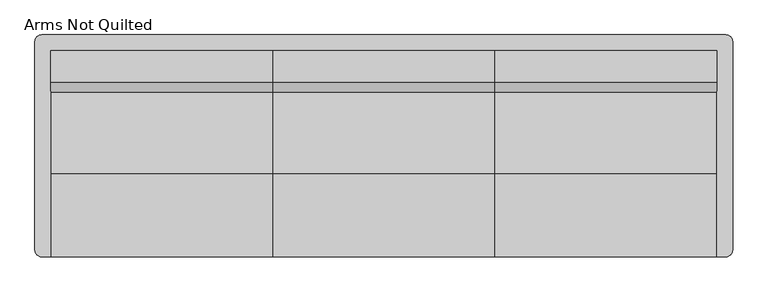
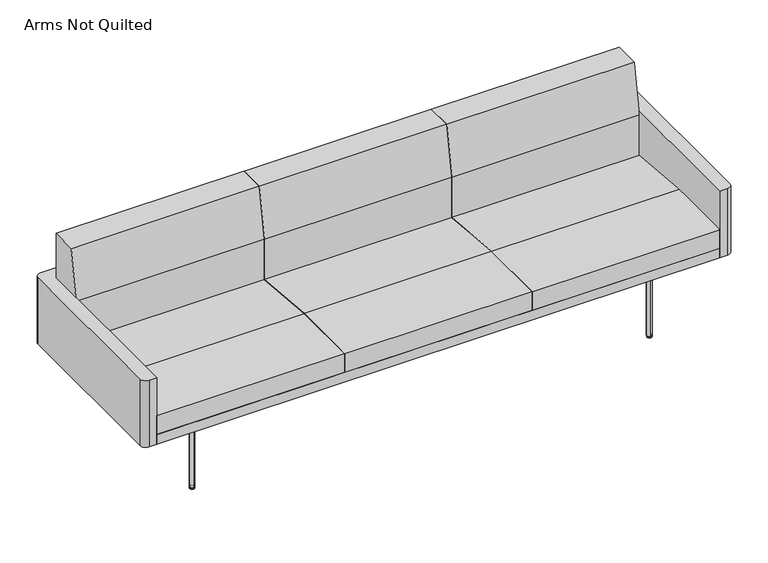
"""IFC4 building model written with IfcOpenShell, lengths in millimetres: furniture geometry, HermanMiller_Collection_Tuxedo_Sofa : Arms Not Quilted."""

from ifc_helpers import new_model, si_unit, point, frame, frame_2d, origin, place, context, project, spatial, polyline, circle_curve, ellipse_curve, trimmed, segment, composite_curve, outline, extrude, source, transform, mapped, element, save
from ifc_brep_helpers import plane_surface, revolved_surface, advanced_brep


def arms_not_quilted_5b6e58a6(model_context):
    return source(origin(), model_context, "Body", "SolidModel", [
        extrude(outline(polyline([(172.790312, 570.0407405), (204.8303749, 761.9999879), (305.047338, 761.9999879), (305.047338, 357.1875), (172.790312, 357.1875), (172.790312, 570.0407405)])), frame((355.8486449, 0.0, 0.0), z_axis=(1.0, 0.0, 0.0), x_axis=(0.0, 1.0, 0.0)), (0.0, 0.0, 1.0), 711.3174324),
        extrude(outline(polyline([(204.8303749, 761.9999879), (305.047338, 761.9999879), (305.047338, 357.1875), (172.790312, 357.1875), (172.790312, 570.0407405), (204.8303749, 761.9999879)])), frame((-1067.1660773, 0.0, 0.0), z_axis=(1.0, 0.0, 0.0), x_axis=(0.0, 1.0, 0.0)), (0.0, 0.0, 1.0), 711.3174324),
        extrude(outline(polyline([(172.790312, 570.0407405), (204.8303749, 761.9999879), (305.047338, 761.9999879), (305.047338, 357.1875), (172.790312, 357.1875), (172.790312, 570.0407405)])), frame((-354.5786449, 0.0, 0.0), z_axis=(1.0, 0.0, 0.0), x_axis=(0.0, 1.0, 0.0)), (0.0, 0.0, 1.0), 709.1572898),
        extrude(outline(polyline([(-355.847338, 357.1875), (-355.847338, 431.3641497), (-89.4717005, 431.3641497), (172.790312, 408.4192229), (172.790312, 357.1875), (-355.847338, 357.1875)])), frame((355.8486449, 0.0, 0.0), z_axis=(1.0, 0.0, 0.0), x_axis=(0.0, 1.0, 0.0)), (0.0, 0.0, 1.0), 711.3174324),
        extrude(outline(polyline([(-355.847338, 431.3641497), (-89.4717005, 431.3641497), (172.790312, 408.4192229), (172.790312, 357.1875), (-355.847338, 357.1875), (-355.847338, 431.3641497)])), frame((-1067.1660773, 0.0, 0.0), z_axis=(1.0, 0.0, 0.0), x_axis=(0.0, 1.0, 0.0)), (0.0, 0.0, 1.0), 711.3174324),
        extrude(outline(polyline([(-355.847338, 357.1875), (-355.847338, 431.3641497), (-89.4717005, 431.3641497), (172.790312, 408.4192229), (172.790312, 357.1875), (-355.847338, 357.1875)])), frame((-354.5786449, 0.0, 0.0), z_axis=(1.0, 0.0, 0.0), x_axis=(0.0, 1.0, 0.0)), (0.0, 0.0, 1.0), 709.1572898),
        advanced_brep(
        [(-862.2241883, -239.6951247, 0.0), (-869.7905542, -239.6951247, 0.0), (-866.0073712, -239.6951247, 0.0), (-856.4823712, -239.6951247, 3.1750001), (-875.5323712, -239.6951247, 3.1750001), (-856.351925, -239.6951247, 6.4931848), (-875.6628174, -239.6951247, 6.4931848), (-861.8574966, -239.6951247, 9.5049435), (-870.1572459, -239.6951247, 9.5049435), (-866.0073712, -239.6951247, 9.5049435)],
        [
            (0, 1, circle_curve(frame((-866.0073712, -239.6951247, 0.0), z_axis=(0.0, 0.0, -1.0), x_axis=(-1.0, 0.0, 0.0)), 3.783183)),
            (1, 2),
            (2, 0),
            (1, 0, circle_curve(frame((-866.0073712, -239.6951247, 0.0), z_axis=(0.0, 0.0, -1.0), x_axis=(-1.0, 0.0, 0.0)), 3.783183)),
            (3, 4, circle_curve(frame((-866.0073712, -239.6951247, 3.1750001), z_axis=(0.0, 0.0, -1.0), x_axis=(-1.0, 0.0, 0.0)), 9.525)),
            (4, 1, circle_curve(frame((-869.7905542, -239.6951247, 6.7793838), z_axis=(0.0, -1.0, 0.0), x_axis=(-1.0, 0.0, 0.0)), 6.7793838)),
            (0, 3, circle_curve(frame((-862.2241883, -239.6951247, 6.7793838), z_axis=(0.0, -1.0, 0.0), x_axis=(1.0, 0.0, 0.0)), 6.7793838)),
            (4, 3, circle_curve(frame((-866.0073712, -239.6951247, 3.1750001), z_axis=(0.0, 0.0, -1.0), x_axis=(-1.0, 0.0, 0.0)), 9.525)),
            (5, 6, circle_curve(frame((-866.0073712, -239.6951247, 6.4931848), z_axis=(0.0, 0.0, -1.0), x_axis=(-1.0, 0.0, 0.0)), 9.6554462)),
            (6, 4),
            (3, 5),
            (6, 5, circle_curve(frame((-866.0073712, -239.6951247, 6.4931848), z_axis=(0.0, 0.0, -1.0), x_axis=(-1.0, 0.0, 0.0)), 9.6554462)),
            (7, 8, circle_curve(frame((-866.0073712, -239.6951247, 9.5049435), z_axis=(0.0, 0.0, -1.0), x_axis=(-1.0, 0.0, 0.0)), 4.1498747)),
            (8, 6, circle_curve(frame((-870.1572459, -239.6951247, 2.9669016), z_axis=(0.0, -1.0, 0.0), x_axis=(-1.0, 0.0, 0.0)), 6.5380418)),
            (5, 7, circle_curve(frame((-861.8574966, -239.6951247, 2.9669016), z_axis=(0.0, -1.0, 0.0), x_axis=(1.0, 0.0, 0.0)), 6.5380418)),
            (8, 7, circle_curve(frame((-866.0073712, -239.6951247, 9.5049435), z_axis=(0.0, 0.0, -1.0), x_axis=(-1.0, 0.0, 0.0)), 4.1498747)),
            (9, 8),
            (7, 9),
        ],
        [
            plane_surface(frame((-866.0073712, -239.6951247, 0.0), z_axis=(0.0, 0.0, -1.0), x_axis=(-1.0, 0.0, 0.0))),
            revolved_surface(trimmed(ellipse_curve(frame((-869.7905542, -239.6951247, 6.7793838), z_axis=(0.0, 1.0, 0.0), x_axis=(-1.0, 0.0, 0.0)), 6.7793838, 6.7793838), [point((-869.7905542, -239.6951247, 0.0))], [point((-875.5323712, -239.6951247, 3.1750001))], True, "CARTESIAN"), (-866.0073712, -239.6951247, 2.4865786), (0.0, 0.0, 1.0)),
            revolved_surface(polyline([(-875.5323712, -239.6951247, 3.1750001), (-875.6628174, -239.6951247, 6.4931848)]), (-866.0073712, -239.6951247, 2.4865786), (0.0, 0.0, 1.0)),
            revolved_surface(trimmed(ellipse_curve(frame((-870.1572459, -239.6951247, 2.9669016), z_axis=(0.0, 1.0, 0.0), x_axis=(-1.0, 0.0, 0.0)), 6.5380418, 6.5380418), [point((-875.6628174, -239.6951247, 6.4931848))], [point((-870.1572459, -239.6951247, 9.5049435))], True, "CARTESIAN"), (-866.0073712, -239.6951247, 2.4865786), (0.0, 0.0, 1.0)),
            plane_surface(frame((-866.0073712, -239.6951247, 9.5049435), z_axis=(0.0, 0.0, 1.0), x_axis=(-1.0, 0.0, 0.0))),
        ],
        [
            (0, [[1, 2, 3]]),
            (0, [[4, -3, -2]]),
            (1, [[5, 6, -1, 7]]),
            (1, [[8, -7, -4, -6]]),
            (2, [[9, 10, -5, 11]]),
            (2, [[12, -11, -8, -10]]),
            (3, [[13, 14, -9, 15]]),
            (3, [[16, -15, -12, -14]]),
            (4, [[17, -13, 18]]),
            (4, [[-18, -16, -17]]),
        ],
    ),
        advanced_brep(
        [(-866.0073712, 332.5700088, 0.0), (-869.7905542, 332.5700088, 0.0), (-862.2241883, 332.5700088, 0.0), (-875.5323712, 332.5700088, 3.1750001), (-856.4823712, 332.5700088, 3.1750001), (-875.6628174, 332.5700088, 6.4931848), (-856.351925, 332.5700088, 6.4931848), (-870.1572459, 332.5700088, 9.5049435), (-861.8574966, 332.5700088, 9.5049435), (-866.0073712, 332.5700088, 9.5049435)],
        [
            (0, 1),
            (1, 2, circle_curve(frame((-866.0073712, 332.5700088, 0.0), z_axis=(0.0, 0.0, -1.0), x_axis=(-1.0, 0.0, 0.0)), 3.783183)),
            (2, 0),
            (2, 1, circle_curve(frame((-866.0073712, 332.5700088, 0.0), z_axis=(0.0, 0.0, -1.0), x_axis=(-1.0, 0.0, 0.0)), 3.783183)),
            (1, 3, circle_curve(frame((-869.7905542, 332.5700088, 6.7793838), z_axis=(0.0, 1.0, 0.0), x_axis=(-1.0, 0.0, 0.0)), 6.7793838)),
            (3, 4, circle_curve(frame((-866.0073712, 332.5700088, 3.1750001), z_axis=(0.0, 0.0, -1.0), x_axis=(-1.0, 0.0, 0.0)), 9.525)),
            (4, 2, circle_curve(frame((-862.2241883, 332.5700088, 6.7793838), z_axis=(0.0, 1.0, 0.0), x_axis=(1.0, 0.0, 0.0)), 6.7793838)),
            (4, 3, circle_curve(frame((-866.0073712, 332.5700088, 3.1750001), z_axis=(0.0, 0.0, -1.0), x_axis=(-1.0, 0.0, 0.0)), 9.525)),
            (3, 5),
            (5, 6, circle_curve(frame((-866.0073712, 332.5700088, 6.4931848), z_axis=(0.0, 0.0, -1.0), x_axis=(-1.0, 0.0, 0.0)), 9.6554462)),
            (6, 4),
            (6, 5, circle_curve(frame((-866.0073712, 332.5700088, 6.4931848), z_axis=(0.0, 0.0, -1.0), x_axis=(-1.0, 0.0, 0.0)), 9.6554462)),
            (5, 7, circle_curve(frame((-870.1572459, 332.5700088, 2.9669016), z_axis=(0.0, 1.0, 0.0), x_axis=(-1.0, 0.0, 0.0)), 6.5380418)),
            (7, 8, circle_curve(frame((-866.0073712, 332.5700088, 9.5049435), z_axis=(0.0, 0.0, -1.0), x_axis=(-1.0, 0.0, 0.0)), 4.1498747)),
            (8, 6, circle_curve(frame((-861.8574966, 332.5700088, 2.9669016), z_axis=(0.0, 1.0, 0.0), x_axis=(1.0, 0.0, 0.0)), 6.5380418)),
            (8, 7, circle_curve(frame((-866.0073712, 332.5700088, 9.5049435), z_axis=(0.0, 0.0, -1.0), x_axis=(-1.0, 0.0, 0.0)), 4.1498747)),
            (7, 9),
            (9, 8),
        ],
        [
            plane_surface(frame((-866.0073712, 332.5700088, 0.0), z_axis=(0.0, 0.0, -1.0), x_axis=(-1.0, 0.0, 0.0))),
            revolved_surface(trimmed(ellipse_curve(frame((-869.7905542, 332.5700088, 6.7793838), z_axis=(0.0, -1.0, 0.0), x_axis=(-1.0, 0.0, 0.0)), 6.7793838, 6.7793838), [point((-875.5323712, 332.5700088, 3.1750001))], [point((-869.7905542, 332.5700088, 0.0))], True, "CARTESIAN"), (-866.0073712, 332.5700088, 2.4865786), (0.0, 0.0, -1.0)),
            revolved_surface(polyline([(-875.6628174, 332.5700088, 6.4931848), (-875.5323712, 332.5700088, 3.1750001)]), (-866.0073712, 332.5700088, 2.4865786), (0.0, 0.0, -1.0)),
            revolved_surface(trimmed(ellipse_curve(frame((-870.1572459, 332.5700088, 2.9669016), z_axis=(0.0, -1.0, 0.0), x_axis=(-1.0, 0.0, 0.0)), 6.5380418, 6.5380418), [point((-870.1572459, 332.5700088, 9.5049435))], [point((-875.6628174, 332.5700088, 6.4931848))], True, "CARTESIAN"), (-866.0073712, 332.5700088, 2.4865786), (0.0, 0.0, -1.0)),
            plane_surface(frame((-866.0073712, 332.5700088, 9.5049435), z_axis=(0.0, 0.0, 1.0), x_axis=(-1.0, 0.0, 0.0))),
        ],
        [
            (0, [[1, 2, 3]]),
            (0, [[-3, 4, -1]]),
            (1, [[-2, 5, 6, 7]]),
            (1, [[-4, -7, 8, -5]]),
            (2, [[-6, 9, 10, 11]]),
            (2, [[-8, -11, 12, -9]]),
            (3, [[-10, 13, 14, 15]]),
            (3, [[-12, -15, 16, -13]]),
            (4, [[-14, 17, 18]]),
            (4, [[-16, -18, -17]]),
        ],
    ),
        extrude(outline(composite_curve([segment(trimmed(circle_curve(frame_2d((-1095.9950773, 333.876338)), 21.971), [point((-1117.9660773, 333.876338))], [point((-1095.9950773, 355.847338))], False, "CARTESIAN"), True, "CONTINUOUS"), segment(polyline([(-1095.9950773, 355.847338), (1095.9950773, 355.847338)]), True, "CONTINUOUS"), segment(trimmed(circle_curve(frame_2d((1095.9950773, 333.876338)), 21.971), [point((1095.9950773, 355.847338))], [point((1117.9660773, 333.876338))], False, "CARTESIAN"), True, "CONTINUOUS"), segment(polyline([(1117.9660773, 333.876338), (1117.9660773, -333.880734)]), True, "CONTINUOUS"), segment(trimmed(circle_curve(frame_2d((1095.9994733, -333.880734)), 21.966604), [point((1117.9660773, -333.880734))], [point((1095.9994733, -355.847338))], False, "CARTESIAN"), True, "CONTINUOUS"), segment(polyline([(1095.9994733, -355.847338), (1067.1660773, -355.847338), (1067.1660773, 305.047338), (-1067.1660773, 305.047338), (-1067.1660773, -355.847338), (-1095.9950773, -355.847338)]), True, "CONTINUOUS"), segment(trimmed(circle_curve(frame_2d((-1095.9950773, -333.876338)), 21.971), [point((-1095.9950773, -355.847338))], [point((-1117.9660773, -333.876338))], False, "CARTESIAN"), True, "CONTINUOUS"), segment(polyline([(-1117.9660773, -333.876338), (-1117.9660773, 333.876338)]), True, "CONTINUOUS")], self_intersect=False)), frame((0.0, 0.0, 317.4993339), z_axis=(0.0, 0.0, 1.0), x_axis=(1.0, 0.0, 0.0)), (0.0, 0.0, 1.0), 266.700654),
        extrude(outline(composite_curve([segment(trimmed(circle_curve(frame_2d((-865.5330732, 332.8903279)), 9.525), [point((-875.0580732, 332.8903279))], [point((-865.5330732, 342.4153279))], False, "CARTESIAN"), True, "CONTINUOUS"), segment(trimmed(circle_curve(frame_2d((-865.5330732, 332.8903279)), 9.525), [point((-865.5330732, 342.4153279))], [point((-856.0080732, 332.8903279))], False, "CARTESIAN"), True, "CONTINUOUS"), segment(trimmed(circle_curve(frame_2d((-865.5330732, 332.8903279)), 9.525), [point((-856.0080732, 332.8903279))], [point((-865.5330732, 323.3653279))], False, "CARTESIAN"), True, "CONTINUOUS"), segment(trimmed(circle_curve(frame_2d((-865.5330732, 332.8903279)), 9.525), [point((-865.5330732, 323.3653279))], [point((-875.0580732, 332.8903279))], False, "CARTESIAN"), True, "CONTINUOUS")], self_intersect=False)), frame((0.0, 0.0, 9.525), z_axis=(0.0, 0.0, 1.0), x_axis=(1.0, 0.0, 0.0)), (0.0, 0.0, 1.0), 269.8750061),
        extrude(outline(composite_curve([segment(trimmed(circle_curve(frame_2d((-865.4343312, -238.7745677)), 9.525), [point((-874.9593312, -238.7745677))], [point((-865.4343312, -229.2495677))], False, "CARTESIAN"), True, "CONTINUOUS"), segment(trimmed(circle_curve(frame_2d((-865.4343312, -238.7745677)), 9.525), [point((-865.4343312, -229.2495677))], [point((-855.9093312, -238.7745677))], False, "CARTESIAN"), True, "CONTINUOUS"), segment(trimmed(circle_curve(frame_2d((-865.4343312, -238.7745677)), 9.525), [point((-855.9093312, -238.7745677))], [point((-865.4343312, -248.2995677))], False, "CARTESIAN"), True, "CONTINUOUS"), segment(trimmed(circle_curve(frame_2d((-865.4343312, -238.7745677)), 9.525), [point((-865.4343312, -248.2995677))], [point((-874.9593312, -238.7745677))], False, "CARTESIAN"), True, "CONTINUOUS")], self_intersect=False)), frame((0.0, 0.0, 9.525), z_axis=(0.0, 0.0, 1.0), x_axis=(1.0, 0.0, 0.0)), (0.0, 0.0, 1.0), 269.8750061),
        advanced_brep(
        [(-861.749631, -238.459695, 0.0), (-869.3159969, -238.459695, 0.0), (-865.532814, -238.459695, 0.0), (-856.007814, -238.459695, 3.1750001), (-875.057814, -238.459695, 3.1750001), (-855.8773678, -238.459695, 6.4931848), (-875.1882602, -238.459695, 6.4931848), (-861.3829393, -238.459695, 9.5049435), (-869.6826886, -238.459695, 9.5049435), (-865.532814, -238.459695, 9.5049435)],
        [
            (0, 1, circle_curve(frame((-865.532814, -238.459695, 0.0), z_axis=(0.0, 0.0, -1.0), x_axis=(-1.0, 0.0, 0.0)), 3.783183)),
            (1, 2),
            (2, 0),
            (1, 0, circle_curve(frame((-865.532814, -238.459695, 0.0), z_axis=(0.0, 0.0, -1.0), x_axis=(-1.0, 0.0, 0.0)), 3.783183)),
            (3, 4, circle_curve(frame((-865.532814, -238.459695, 3.1750001), z_axis=(0.0, 0.0, -1.0), x_axis=(-1.0, 0.0, 0.0)), 9.525)),
            (4, 1, circle_curve(frame((-869.3159969, -238.459695, 6.7793838), z_axis=(0.0, -1.0, 0.0), x_axis=(-1.0, 0.0, 0.0)), 6.7793838)),
            (0, 3, circle_curve(frame((-861.749631, -238.459695, 6.7793838), z_axis=(0.0, -1.0, 0.0), x_axis=(1.0, 0.0, 0.0)), 6.7793838)),
            (4, 3, circle_curve(frame((-865.532814, -238.459695, 3.1750001), z_axis=(0.0, 0.0, -1.0), x_axis=(-1.0, 0.0, 0.0)), 9.525)),
            (5, 6, circle_curve(frame((-865.532814, -238.459695, 6.4931848), z_axis=(0.0, 0.0, -1.0), x_axis=(-1.0, 0.0, 0.0)), 9.6554462)),
            (6, 4),
            (3, 5),
            (6, 5, circle_curve(frame((-865.532814, -238.459695, 6.4931848), z_axis=(0.0, 0.0, -1.0), x_axis=(-1.0, 0.0, 0.0)), 9.6554462)),
            (7, 8, circle_curve(frame((-865.532814, -238.459695, 9.5049435), z_axis=(0.0, 0.0, -1.0), x_axis=(-1.0, 0.0, 0.0)), 4.1498747)),
            (8, 6, circle_curve(frame((-869.6826886, -238.459695, 2.9669016), z_axis=(0.0, -1.0, 0.0), x_axis=(-1.0, 0.0, 0.0)), 6.5380418)),
            (5, 7, circle_curve(frame((-861.3829393, -238.459695, 2.9669016), z_axis=(0.0, -1.0, 0.0), x_axis=(1.0, 0.0, 0.0)), 6.5380418)),
            (8, 7, circle_curve(frame((-865.532814, -238.459695, 9.5049435), z_axis=(0.0, 0.0, -1.0), x_axis=(-1.0, 0.0, 0.0)), 4.1498747)),
            (9, 8),
            (7, 9),
        ],
        [
            plane_surface(frame((-865.532814, -238.459695, 0.0), z_axis=(0.0, 0.0, -1.0), x_axis=(-1.0, 0.0, 0.0))),
            revolved_surface(trimmed(ellipse_curve(frame((-869.3159969, -238.459695, 6.7793838), z_axis=(0.0, 1.0, 0.0), x_axis=(-1.0, 0.0, 0.0)), 6.7793838, 6.7793838), [point((-869.3159969, -238.459695, 0.0))], [point((-875.057814, -238.459695, 3.1750001))], True, "CARTESIAN"), (-865.532814, -238.459695, 2.4865786), (0.0, 0.0, 1.0)),
            revolved_surface(polyline([(-875.057814, -238.459695, 3.1750001), (-875.1882602, -238.459695, 6.4931848)]), (-865.532814, -238.459695, 2.4865786), (0.0, 0.0, 1.0)),
            revolved_surface(trimmed(ellipse_curve(frame((-869.6826886, -238.459695, 2.9669016), z_axis=(0.0, 1.0, 0.0), x_axis=(-1.0, 0.0, 0.0)), 6.5380418, 6.5380418), [point((-875.1882602, -238.459695, 6.4931848))], [point((-869.6826886, -238.459695, 9.5049435))], True, "CARTESIAN"), (-865.532814, -238.459695, 2.4865786), (0.0, 0.0, 1.0)),
            plane_surface(frame((-865.532814, -238.459695, 9.5049435), z_axis=(0.0, 0.0, 1.0), x_axis=(-1.0, 0.0, 0.0))),
        ],
        [
            (0, [[1, 2, 3]]),
            (0, [[4, -3, -2]]),
            (1, [[5, 6, -1, 7]]),
            (1, [[8, -7, -4, -6]]),
            (2, [[9, 10, -5, 11]]),
            (2, [[12, -11, -8, -10]]),
            (3, [[13, 14, -9, 15]]),
            (3, [[16, -15, -12, -14]]),
            (4, [[17, -13, 18]]),
            (4, [[-18, -16, -17]]),
        ],
    ),
        advanced_brep(
        [(-865.8408432, 332.7425888, 0.0), (-869.6240261, 332.7425888, 0.0), (-862.0576602, 332.7425888, 0.0), (-875.3658432, 332.7425888, 3.1750001), (-856.3158432, 332.7425888, 3.1750001), (-875.4962893, 332.7425888, 6.4931848), (-856.185397, 332.7425888, 6.4931848), (-869.9907178, 332.7425888, 9.5049435), (-861.6909685, 332.7425888, 9.5049435), (-865.8408432, 332.7425888, 9.5049435)],
        [
            (0, 1),
            (1, 2, circle_curve(frame((-865.8408432, 332.7425888, 0.0), z_axis=(0.0, 0.0, -1.0), x_axis=(-1.0, 0.0, 0.0)), 3.783183)),
            (2, 0),
            (2, 1, circle_curve(frame((-865.8408432, 332.7425888, 0.0), z_axis=(0.0, 0.0, -1.0), x_axis=(-1.0, 0.0, 0.0)), 3.783183)),
            (1, 3, circle_curve(frame((-869.6240261, 332.7425888, 6.7793838), z_axis=(0.0, 1.0, 0.0), x_axis=(-1.0, 0.0, 0.0)), 6.7793838)),
            (3, 4, circle_curve(frame((-865.8408432, 332.7425888, 3.1750001), z_axis=(0.0, 0.0, -1.0), x_axis=(-1.0, 0.0, 0.0)), 9.525)),
            (4, 2, circle_curve(frame((-862.0576602, 332.7425888, 6.7793838), z_axis=(0.0, 1.0, 0.0), x_axis=(1.0, 0.0, 0.0)), 6.7793838)),
            (4, 3, circle_curve(frame((-865.8408432, 332.7425888, 3.1750001), z_axis=(0.0, 0.0, -1.0), x_axis=(-1.0, 0.0, 0.0)), 9.525)),
            (3, 5),
            (5, 6, circle_curve(frame((-865.8408432, 332.7425888, 6.4931848), z_axis=(0.0, 0.0, -1.0), x_axis=(-1.0, 0.0, 0.0)), 9.6554462)),
            (6, 4),
            (6, 5, circle_curve(frame((-865.8408432, 332.7425888, 6.4931848), z_axis=(0.0, 0.0, -1.0), x_axis=(-1.0, 0.0, 0.0)), 9.6554462)),
            (5, 7, circle_curve(frame((-869.9907178, 332.7425888, 2.9669016), z_axis=(0.0, 1.0, 0.0), x_axis=(-1.0, 0.0, 0.0)), 6.5380418)),
            (7, 8, circle_curve(frame((-865.8408432, 332.7425888, 9.5049435), z_axis=(0.0, 0.0, -1.0), x_axis=(-1.0, 0.0, 0.0)), 4.1498747)),
            (8, 6, circle_curve(frame((-861.6909685, 332.7425888, 2.9669016), z_axis=(0.0, 1.0, 0.0), x_axis=(1.0, 0.0, 0.0)), 6.5380418)),
            (8, 7, circle_curve(frame((-865.8408432, 332.7425888, 9.5049435), z_axis=(0.0, 0.0, -1.0), x_axis=(-1.0, 0.0, 0.0)), 4.1498747)),
            (7, 9),
            (9, 8),
        ],
        [
            plane_surface(frame((-865.8408432, 332.7425888, 0.0), z_axis=(0.0, 0.0, -1.0), x_axis=(-1.0, 0.0, 0.0))),
            revolved_surface(trimmed(ellipse_curve(frame((-869.6240261, 332.7425888, 6.7793838), z_axis=(0.0, -1.0, 0.0), x_axis=(-1.0, 0.0, 0.0)), 6.7793838, 6.7793838), [point((-875.3658432, 332.7425888, 3.1750001))], [point((-869.6240261, 332.7425888, 0.0))], True, "CARTESIAN"), (-865.8408432, 332.7425888, 2.4865786), (0.0, 0.0, -1.0)),
            revolved_surface(polyline([(-875.4962893, 332.7425888, 6.4931848), (-875.3658432, 332.7425888, 3.1750001)]), (-865.8408432, 332.7425888, 2.4865786), (0.0, 0.0, -1.0)),
            revolved_surface(trimmed(ellipse_curve(frame((-869.9907178, 332.7425888, 2.9669016), z_axis=(0.0, -1.0, 0.0), x_axis=(-1.0, 0.0, 0.0)), 6.5380418, 6.5380418), [point((-869.9907178, 332.7425888, 9.5049435))], [point((-875.4962893, 332.7425888, 6.4931848))], True, "CARTESIAN"), (-865.8408432, 332.7425888, 2.4865786), (0.0, 0.0, -1.0)),
            plane_surface(frame((-865.8408432, 332.7425888, 9.5049435), z_axis=(0.0, 0.0, 1.0), x_axis=(-1.0, 0.0, 0.0))),
        ],
        [
            (0, [[1, 2, 3]]),
            (0, [[-3, 4, -1]]),
            (1, [[-2, 5, 6, 7]]),
            (1, [[-4, -7, 8, -5]]),
            (2, [[-6, 9, 10, 11]]),
            (2, [[-8, -11, 12, -9]]),
            (3, [[-10, 13, 14, 15]]),
            (3, [[-12, -15, 16, -13]]),
            (4, [[-14, 17, 18]]),
            (4, [[-16, -18, -17]]),
        ],
    ),
        advanced_brep(
        [(867.9917462, -239.6951247, 0.0), (871.7749292, -239.6951247, 0.0), (864.2085633, -239.6951247, 0.0), (877.5167462, -239.6951247, 3.1750001), (858.4667462, -239.6951247, 3.1750001), (877.6471924, -239.6951247, 6.4931848), (858.3363, -239.6951247, 6.4931848), (872.1416209, -239.6951247, 9.5049434), (863.8418716, -239.6951247, 9.5049434), (867.9917462, -239.6951247, 9.5049435)],
        [
            (0, 1),
            (1, 2, circle_curve(frame((867.9917462, -239.6951247, 0.0), z_axis=(0.0, 0.0, -1.0), x_axis=(1.0, 0.0, 0.0)), 3.783183)),
            (2, 0),
            (2, 1, circle_curve(frame((867.9917462, -239.6951247, 0.0), z_axis=(0.0, 0.0, -1.0), x_axis=(1.0, 0.0, 0.0)), 3.783183)),
            (1, 3, circle_curve(frame((871.7749292, -239.6951247, 6.7793838), z_axis=(0.0, -1.0, 0.0), x_axis=(1.0, 0.0, 0.0)), 6.7793838)),
            (3, 4, circle_curve(frame((867.9917462, -239.6951247, 3.1750001), z_axis=(0.0, 0.0, -1.0), x_axis=(1.0, 0.0, 0.0)), 9.525)),
            (4, 2, circle_curve(frame((864.2085633, -239.6951247, 6.7793838), z_axis=(0.0, -1.0, 0.0), x_axis=(-1.0, 0.0, 0.0)), 6.7793838)),
            (4, 3, circle_curve(frame((867.9917462, -239.6951247, 3.1750001), z_axis=(0.0, 0.0, -1.0), x_axis=(1.0, 0.0, 0.0)), 9.525)),
            (3, 5),
            (5, 6, circle_curve(frame((867.9917462, -239.6951247, 6.4931848), z_axis=(0.0, 0.0, -1.0), x_axis=(1.0, 0.0, 0.0)), 9.6554462)),
            (6, 4),
            (6, 5, circle_curve(frame((867.9917462, -239.6951247, 6.4931848), z_axis=(0.0, 0.0, -1.0), x_axis=(1.0, 0.0, 0.0)), 9.6554462)),
            (5, 7, circle_curve(frame((872.1416209, -239.6951247, 2.9669016), z_axis=(0.0, -1.0, 0.0), x_axis=(1.0, 0.0, 0.0)), 6.5380418)),
            (7, 8, circle_curve(frame((867.9917462, -239.6951247, 9.5049434), z_axis=(0.0, 0.0, -1.0), x_axis=(1.0, 0.0, 0.0)), 4.1498747)),
            (8, 6, circle_curve(frame((863.8418716, -239.6951247, 2.9669016), z_axis=(0.0, -1.0, 0.0), x_axis=(-1.0, 0.0, 0.0)), 6.5380418)),
            (8, 7, circle_curve(frame((867.9917462, -239.6951247, 9.5049434), z_axis=(0.0, 0.0, -1.0), x_axis=(1.0, 0.0, 0.0)), 4.1498747)),
            (7, 9),
            (9, 8),
        ],
        [
            plane_surface(frame((867.9917462, -239.6951247, 0.0), z_axis=(0.0, 0.0, -1.0), x_axis=(1.0, 0.0, 0.0))),
            revolved_surface(trimmed(ellipse_curve(frame((871.7749292, -239.6951247, 6.7793838), z_axis=(0.0, 1.0, 0.0), x_axis=(1.0, 0.0, 0.0)), 6.7793838, 6.7793838), [point((877.5167462, -239.6951247, 3.1750001))], [point((871.7749292, -239.6951247, 0.0))], True, "CARTESIAN"), (867.9917462, -239.6951247, 2.4865786), (0.0, 0.0, -1.0)),
            revolved_surface(polyline([(877.6471924, -239.6951247, 6.4931848), (877.5167462, -239.6951247, 3.1750001)]), (867.9917462, -239.6951247, 2.4865786), (0.0, 0.0, -1.0)),
            revolved_surface(trimmed(ellipse_curve(frame((872.1416209, -239.6951247, 2.9669016), z_axis=(0.0, 1.0, 0.0), x_axis=(1.0, 0.0, 0.0)), 6.5380418, 6.5380418), [point((872.1416209, -239.6951247, 9.5049434))], [point((877.6471924, -239.6951247, 6.4931848))], True, "CARTESIAN"), (867.9917462, -239.6951247, 2.4865786), (0.0, 0.0, -1.0)),
            plane_surface(frame((867.9917462, -239.6951247, 9.5049435), z_axis=(0.0, 0.0, 1.0), x_axis=(1.0, 0.0, 0.0))),
        ],
        [
            (0, [[1, 2, 3]]),
            (0, [[-3, 4, -1]]),
            (1, [[-2, 5, 6, 7]]),
            (1, [[-4, -7, 8, -5]]),
            (2, [[-6, 9, 10, 11]]),
            (2, [[-8, -11, 12, -9]]),
            (3, [[-10, 13, 14, 15]]),
            (3, [[-12, -15, 16, -13]]),
            (4, [[-14, 17, 18]]),
            (4, [[-16, -18, -17]]),
        ],
    ),
        advanced_brep(
        [(864.2085633, 332.5700088, 0.0), (871.7749292, 332.5700088, 0.0), (867.9917462, 332.5700088, 0.0), (858.4667462, 332.5700088, 3.1750001), (877.5167462, 332.5700088, 3.1750001), (858.3363, 332.5700088, 6.4931848), (877.6471924, 332.5700088, 6.4931848), (863.8418716, 332.5700088, 9.5049435), (872.1416209, 332.5700088, 9.5049435), (867.9917462, 332.5700088, 9.5049435)],
        [
            (0, 1, circle_curve(frame((867.9917462, 332.5700088, 0.0), z_axis=(0.0, 0.0, -1.0), x_axis=(1.0, 0.0, 0.0)), 3.783183)),
            (1, 2),
            (2, 0),
            (1, 0, circle_curve(frame((867.9917462, 332.5700088, 0.0), z_axis=(0.0, 0.0, -1.0), x_axis=(1.0, 0.0, 0.0)), 3.783183)),
            (3, 4, circle_curve(frame((867.9917462, 332.5700088, 3.1750001), z_axis=(0.0, 0.0, -1.0), x_axis=(1.0, 0.0, 0.0)), 9.525)),
            (4, 1, circle_curve(frame((871.7749292, 332.5700088, 6.7793838), z_axis=(0.0, 1.0, 0.0), x_axis=(1.0, 0.0, 0.0)), 6.7793838)),
            (0, 3, circle_curve(frame((864.2085633, 332.5700088, 6.7793838), z_axis=(0.0, 1.0, 0.0), x_axis=(-1.0, 0.0, 0.0)), 6.7793838)),
            (4, 3, circle_curve(frame((867.9917462, 332.5700088, 3.1750001), z_axis=(0.0, 0.0, -1.0), x_axis=(1.0, 0.0, 0.0)), 9.525)),
            (5, 6, circle_curve(frame((867.9917462, 332.5700088, 6.4931848), z_axis=(0.0, 0.0, -1.0), x_axis=(1.0, 0.0, 0.0)), 9.6554462)),
            (6, 4),
            (3, 5),
            (6, 5, circle_curve(frame((867.9917462, 332.5700088, 6.4931848), z_axis=(0.0, 0.0, -1.0), x_axis=(1.0, 0.0, 0.0)), 9.6554462)),
            (7, 8, circle_curve(frame((867.9917462, 332.5700088, 9.5049435), z_axis=(0.0, 0.0, -1.0), x_axis=(1.0, 0.0, 0.0)), 4.1498747)),
            (8, 6, circle_curve(frame((872.1416209, 332.5700088, 2.9669016), z_axis=(0.0, 1.0, 0.0), x_axis=(1.0, 0.0, 0.0)), 6.5380418)),
            (5, 7, circle_curve(frame((863.8418716, 332.5700088, 2.9669016), z_axis=(0.0, 1.0, 0.0), x_axis=(-1.0, 0.0, 0.0)), 6.5380418)),
            (8, 7, circle_curve(frame((867.9917462, 332.5700088, 9.5049435), z_axis=(0.0, 0.0, -1.0), x_axis=(1.0, 0.0, 0.0)), 4.1498747)),
            (9, 8),
            (7, 9),
        ],
        [
            plane_surface(frame((867.9917462, 332.5700088, 0.0), z_axis=(0.0, 0.0, -1.0), x_axis=(1.0, 0.0, 0.0))),
            revolved_surface(trimmed(ellipse_curve(frame((871.7749292, 332.5700088, 6.7793838), z_axis=(0.0, -1.0, 0.0), x_axis=(1.0, 0.0, 0.0)), 6.7793838, 6.7793838), [point((871.7749292, 332.5700088, 0.0))], [point((877.5167462, 332.5700088, 3.1750001))], True, "CARTESIAN"), (867.9917462, 332.5700088, 2.4865786), (0.0, 0.0, 1.0)),
            revolved_surface(polyline([(877.5167462, 332.5700088, 3.1750001), (877.6471924, 332.5700088, 6.4931848)]), (867.9917462, 332.5700088, 2.4865786), (0.0, 0.0, 1.0)),
            revolved_surface(trimmed(ellipse_curve(frame((872.1416209, 332.5700088, 2.9669016), z_axis=(0.0, -1.0, 0.0), x_axis=(1.0, 0.0, 0.0)), 6.5380418, 6.5380418), [point((877.6471924, 332.5700088, 6.4931848))], [point((872.1416209, 332.5700088, 9.5049435))], True, "CARTESIAN"), (867.9917462, 332.5700088, 2.4865786), (0.0, 0.0, 1.0)),
            plane_surface(frame((867.9917462, 332.5700088, 9.5049435), z_axis=(0.0, 0.0, 1.0), x_axis=(1.0, 0.0, 0.0))),
        ],
        [
            (0, [[1, 2, 3]]),
            (0, [[4, -3, -2]]),
            (1, [[5, 6, -1, 7]]),
            (1, [[8, -7, -4, -6]]),
            (2, [[9, 10, -5, 11]]),
            (2, [[12, -11, -8, -10]]),
            (3, [[13, 14, -9, 15]]),
            (3, [[16, -15, -12, -14]]),
            (4, [[17, -13, 18]]),
            (4, [[-18, -16, -17]]),
        ],
    ),
        extrude(outline(composite_curve([segment(trimmed(circle_curve(frame_2d((867.5174482, 332.8903279)), 9.525), [point((877.0424482, 332.8903279))], [point((867.5174482, 323.3653279))], False, "CARTESIAN"), True, "CONTINUOUS"), segment(trimmed(circle_curve(frame_2d((867.5174482, 332.8903279)), 9.525), [point((867.5174482, 323.3653279))], [point((857.9924482, 332.8903279))], False, "CARTESIAN"), True, "CONTINUOUS"), segment(trimmed(circle_curve(frame_2d((867.5174482, 332.8903279)), 9.525), [point((857.9924482, 332.8903279))], [point((867.5174482, 342.4153279))], False, "CARTESIAN"), True, "CONTINUOUS"), segment(trimmed(circle_curve(frame_2d((867.5174482, 332.8903279)), 9.525), [point((867.5174482, 342.4153279))], [point((877.0424482, 332.8903279))], False, "CARTESIAN"), True, "CONTINUOUS")], self_intersect=False)), frame((0.0, 0.0, 9.525), z_axis=(0.0, 0.0, 1.0), x_axis=(1.0, 0.0, 0.0)), (0.0, 0.0, 1.0), 269.8750061),
        extrude(outline(composite_curve([segment(trimmed(circle_curve(frame_2d((867.4187062, -238.7745677)), 9.525), [point((876.9437062, -238.7745677))], [point((867.4187062, -248.2995677))], False, "CARTESIAN"), True, "CONTINUOUS"), segment(trimmed(circle_curve(frame_2d((867.4187062, -238.7745677)), 9.525), [point((867.4187062, -248.2995677))], [point((857.8937062, -238.7745677))], False, "CARTESIAN"), True, "CONTINUOUS"), segment(trimmed(circle_curve(frame_2d((867.4187062, -238.7745677)), 9.525), [point((857.8937062, -238.7745677))], [point((867.4187062, -229.2495677))], False, "CARTESIAN"), True, "CONTINUOUS"), segment(trimmed(circle_curve(frame_2d((867.4187062, -238.7745677)), 9.525), [point((867.4187062, -229.2495677))], [point((876.9437062, -238.7745677))], False, "CARTESIAN"), True, "CONTINUOUS")], self_intersect=False)), frame((0.0, 0.0, 9.525), z_axis=(0.0, 0.0, 1.0), x_axis=(1.0, 0.0, 0.0)), (0.0, 0.0, 1.0), 269.8750061),
        extrude(outline(polyline([(877.2925536, 342.5689221), (877.2925536, -248.3227239), (-877.2925536, -248.3227239), (-877.2925536, 342.5689221), (877.2925536, 342.5689221)]), holes=[polyline([(858.2425536, 323.5189221), (-858.2425536, 323.5189221), (-858.2425536, -229.2727239), (858.2425536, -229.2727239), (858.2425536, 323.5189221)])]), frame((0.0, 0.0, 279.4000061), z_axis=(0.0, 0.0, 1.0), x_axis=(1.0, 0.0, 0.0)), (0.0, 0.0, 1.0), 38.0999818),
        extrude(outline(polyline([(-1067.1660773, 305.047338), (1067.1660773, 305.047338), (1067.1660773, -355.847338), (-1067.1660773, -355.847338), (-1067.1660773, 305.047338)])), frame((0.0, 0.0, 318.7699879), z_axis=(0.0, 0.0, 1.0), x_axis=(1.0, 0.0, 0.0)), (0.0, 0.0, 1.0), 37.1475121),
    ])


if __name__ == "__main__":
    model = new_model("IFC4")
    model_context = context("Model", 3, world=origin())
    ifc_project = project(units=[si_unit("LENGTHUNIT", "METRE", prefix="MILLI")], contexts=[model_context])
    site = spatial("IfcSite", under=ifc_project)
    building = spatial("IfcBuilding", under=site)
    placement = place(None, origin())
    arms_not_quilted_shape = arms_not_quilted_5b6e58a6(model_context)
    element("IfcFurniture", 1, ObjectType="HermanMiller_Collection_Tuxedo_Sofa : Arms Not Quilted", at=placement, inside=building, context=model_context, shape_type="MappedRepresentation", body=[
        mapped(arms_not_quilted_shape, transform((0.0, 0.0, 0.0), x_axis=(1.0, 0.0, 0.0), y_axis=(0.0, 1.0, 0.0), z_axis=(0.0, 0.0, 1.0))),
    ])
    save(model, "model.ifc")

# Revit data of these elements
# Type "HermanMiller_Collection_Tuxedo_Sofa : Arms Not Quilted"
#   Watermarked By = "http://revitwatermark.com"
#   URL = "http://www.hermanmiller.com\r\n"
#   Product Documentation Link = "http://www.hermanmiller.com/products/seating/lounge-seating/tuxedo-lounge-seating.html"
#   Model = "ST3AN"
#   Manufacturer = "Herman Miller, Inc."
#   Description = "Tuxedo Sofa Arms Not Quilted"
#   Copyright © = "Copyright © Herman Miller, Inc."
#   Catalog Code = "HMH"
#   Catalog = "Herman Miller Collection"
#   Base Price [instance default] = ""
#   Assembly Code = "E2020200"
#   spacing = 0' - 2.91982"
#   quiltLength = 0' - 6.85"
#   quiltHeight = 0' - 3.3"
#   quiltGapHalf = 0' - 0.075"
#   quiltGap = 0' - 0.15"
#   quiltEdgeGap = 0' - 0.83941"
#   quilt Length = 0' - 7"
#   quilt Height = 0' - 3.35"
#   frameThickness = 0' - 0 3/4"
#   cutHeight [instance default] = 0' - 4.4"
#   Arm Thicknes = 0' - 2"
#   Quilted [instance default] = no
#   Package Qty = 1
#   Not Quilted [instance default] = yes
#   Has Arms [instance default] = yes
#   Arms Off [instance default] = no
#   Upholstery [instance default] = Herman Miller - Seat Fabric 8R18 Twist Sepia
#   Base Finish [instance default] = Herman Miller - Finish AS Arctic Silver
#   Type Comments = ""
# Element 1 (IfcFurniture, "HermanMiller_Collection_Tuxedo_Sofa : Arms Not Quilted")
#   Materials on its faces: "Herman Miller - Finish AS Arctic Silver", "Herman Miller - Seat Fabric 8R18 Twist Sepia"
# Materials
#   "Herman Miller - Seat Fabric 8R18 Twist Sepia": class "Unassigned", colour RGB 132 112 87, transparency 0, Keynote = "﻿﻿         ﻿                      ​     ​   ​  ﻿   ​                   ﻿       ﻿   ﻿           ​  ​   ​                ﻿        ﻿  ﻿      ﻿  ﻿      ​     ﻿                       ﻿ ​ ​   ﻿    ​​       ﻿            ﻿﻿﻿﻿               ﻿      ﻿   ﻿﻿​ ﻿         ﻿    ﻿        ​      ​   ﻿  ​ ﻿         ﻿ ​     ﻿                ﻿﻿", Comments = "﻿﻿         ﻿                      ​     ​   ​  ﻿   ​                   ﻿       ﻿   ﻿           ​  ​   ​                ﻿        ﻿  ﻿      ﻿  ﻿      ​     ﻿                       ﻿ ​ ​   ﻿    ​​       ﻿            ﻿﻿﻿﻿               ﻿      ﻿   ﻿﻿​ ﻿         ﻿    ﻿        ​      ​   ﻿  ​ ﻿         ﻿ ​     ﻿                ﻿﻿", Description = "﻿﻿         ﻿                      ​     ​   ​  ﻿   ​                   ﻿       ﻿   ﻿           ​  ​   ​                ﻿        ﻿  ﻿      ﻿  ﻿      ​     ﻿                       ﻿ ​ ​   ﻿    ​​       ﻿            ﻿﻿﻿﻿               ﻿      ﻿   ﻿﻿​ ﻿         ﻿    ﻿        ​      ​   ﻿  ​ ﻿         ﻿ ​     ﻿                ﻿﻿"
#   "Herman Miller - Finish AS Arctic Silver": class "Plastic", colour RGB 188 188 191, transparency 0, Keynote = "﻿﻿         ﻿                      ​     ​   ​  ﻿   ​                   ﻿       ﻿   ﻿           ​  ​   ​                ﻿        ﻿  ﻿      ﻿  ﻿      ​     ﻿                       ﻿ ​ ​   ﻿    ​​       ﻿            ﻿﻿﻿﻿               ﻿      ﻿   ﻿﻿​ ﻿         ﻿    ﻿        ​      ​   ﻿  ​ ﻿         ﻿ ​     ﻿                ﻿﻿", Comments = "﻿﻿         ﻿                      ​     ​   ​  ﻿   ​                   ﻿       ﻿   ﻿           ​  ​   ​                ﻿        ﻿  ﻿      ﻿  ﻿      ​     ﻿                       ﻿ ​ ​   ﻿    ​​       ﻿            ﻿﻿﻿﻿               ﻿      ﻿   ﻿﻿​ ﻿         ﻿    ﻿        ​      ​   ﻿  ​ ﻿         ﻿ ​     ﻿                ﻿﻿", Description = "﻿﻿         ﻿                      ​     ​   ​  ﻿   ​                   ﻿       ﻿   ﻿           ​  ​   ​                ﻿        ﻿  ﻿      ﻿  ﻿      ​     ﻿                       ﻿ ​ ​   ﻿    ​​       ﻿            ﻿﻿﻿﻿               ﻿      ﻿   ﻿﻿​ ﻿         ﻿    ﻿        ​      ​   ﻿  ​ ﻿         ﻿ ​     ﻿                ﻿﻿"
